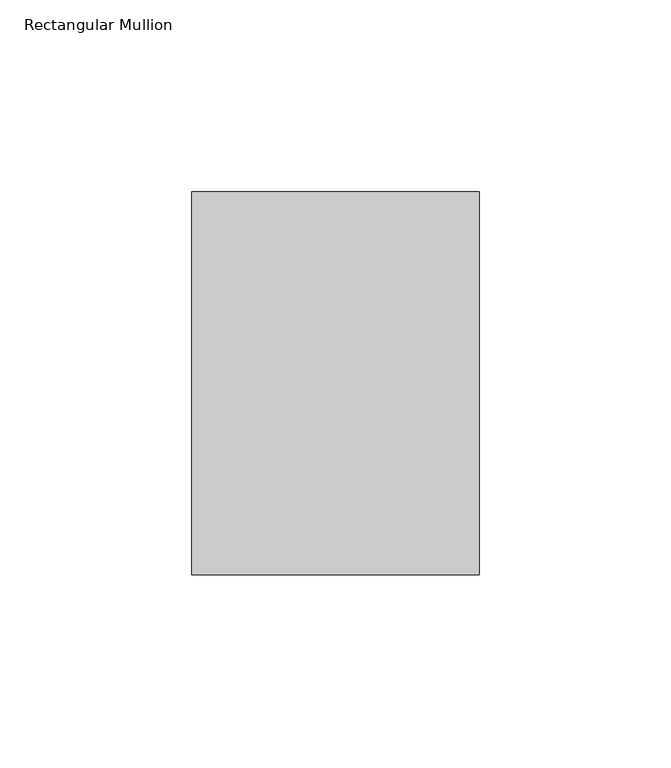
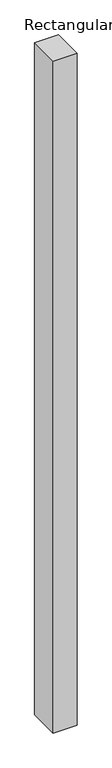
"""IFC4 building model written with IfcOpenShell, lengths in millimetres: member geometry, Rectangular Mullion : 알루미늄_Rectangular Cap_100 x 75."""

from ifc_helpers import new_model, si_unit, frame, origin, place, context, project, spatial, polyline, outline, extrude, source, transform, mapped, element, save


def rectangular_mullion_ea539452(model_context):
    return source(origin(), model_context, "Body", "SweptSolid", [
        extrude(outline(polyline([(0.0, 50.0), (0.0, -50.0), (-75.0, -50.0), (-75.0, 50.0), (0.0, 50.0)])), frame((0.0, 0.0, -2222.5), z_axis=(0.0, 0.0, 1.0), x_axis=(1.0, 0.0, 0.0)), (0.0, 0.0, 1.0), 2222.5),
    ])


if __name__ == "__main__":
    model = new_model("IFC4")
    model_context = context("Model", 3, world=origin())
    ifc_project = project(units=[si_unit("LENGTHUNIT", "METRE", prefix="MILLI")], contexts=[model_context])
    site = spatial("IfcSite", under=ifc_project)
    building = spatial("IfcBuilding", under=site)
    placement = place(None, origin())
    rectangular_mullion_shape = rectangular_mullion_ea539452(model_context)
    element("IfcMember", 1, ObjectType="Rectangular Mullion : 알루미늄_Rectangular Cap_100 x 75", at=placement, inside=building, context=model_context, shape_type="MappedRepresentation", body=[
        mapped(rectangular_mullion_shape, transform((0.0, 0.0, 0.0), x_axis=(1.0, 0.0, 0.0), y_axis=(0.0, 1.0, 0.0), z_axis=(0.0, 0.0, 1.0))),
    ])
    save(model, "model.ifc")

# Revit data of these elements
# Type "Rectangular Mullion : 알루미늄_Rectangular Cap_100 x 75"
#   built-in parameter 1007304 = 0.328084 (stored number, unit not read)
#   built-in parameter 1007301 = 0.123031 (stored number, unit not read)
#   built-in parameter 1007300 = 0.123031 (stored number, unit not read)
# Element 1 (IfcMember, "Rectangular Mullion : 알루미늄_Rectangular Cap_100 x 75")
#   Materials on its faces: "00_Metal_Stainless Steel"
# Materials
#   "00_Metal_Stainless Steel": class "Metal", colour RGB 148 148 148, transparency 0, Description = "Steel", Cost = 0
